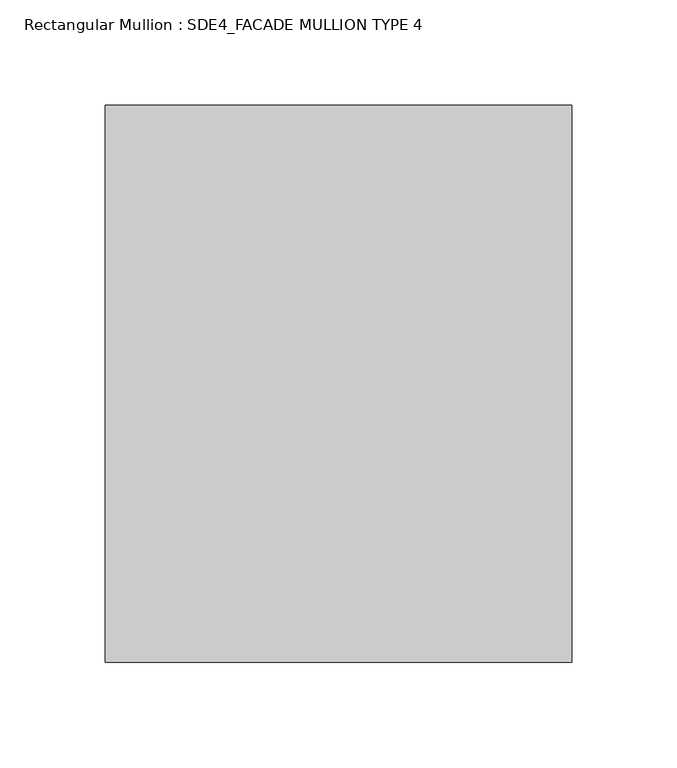
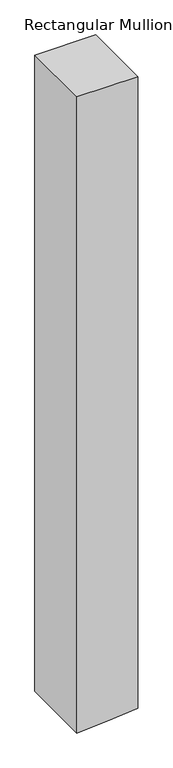
"""IFC4 building model written with IfcOpenShell, lengths in millimetres: member geometry, Rectangular Mullion : SDE4_FACADE MULLION TYPE 4."""

import ifcopenshell
import ifcopenshell.guid

model = None  # the IFC model being written
_history = None  # IfcOwnerHistory: only IFC2X3 demands one
_inside = {}  # id of a spatial element -> (the spatial element, [elements in it])
_under = {}  # id of a project, library or spatial element -> (it, [spatial elements below it])
_declared = {}  # id of a project -> (the project, [libraries it declares])
_typed = {}  # id of a type object -> (the type object, [elements of that type])
_made_of = {}  # id of a material, layer set ... -> (it, [elements and type objects made of it])


def new_model(schema):
    """Start an empty IFC model of exactly this schema.

    Asked for "IFC4X3", IfcOpenShell would pick the latest addendum, in which some entities
    have other attributes; the version numbers below select the first issue.
    IFC2X3 requires an IfcOwnerHistory on every rooted entity: one is made here for all.
    """
    global model, _history
    if schema == "IFC4X3":
        model = ifcopenshell.file(schema_version=(4, 3, 0, 0))
    else:
        model = ifcopenshell.file(schema=schema)
    _inside.clear()
    _under.clear()
    _declared.clear()
    _typed.clear()
    _made_of.clear()
    _history = None
    if model.schema == "IFC2X3":
        org = make("IfcOrganization", Name="unknown")
        user = make(
            "IfcPersonAndOrganization",
            ThePerson=make("IfcPerson", FamilyName="unknown"),
            TheOrganization=org,
        )
        app = make(
            "IfcApplication",
            ApplicationDeveloper=org,
            Version="unknown",
            ApplicationFullName="unknown",
            ApplicationIdentifier="unknown",
        )
        _history = make(
            "IfcOwnerHistory",
            OwningUser=user,
            OwningApplication=app,
            ChangeAction="ADDED",
            CreationDate=0,
        )
    return model


def make(cls, **values):
    """One entity of the class cls with the attributes given. An attribute that is None is left unset."""
    return model.create_entity(
        cls, **{name: value for name, value in values.items() if value is not None}
    )


def rooted(cls, **values):
    """An entity with a GlobalId (a new one), such as an element, a storey or a relation."""
    return make(cls, GlobalId=ifcopenshell.guid.new(), OwnerHistory=_history, **values)


def si_unit(unit_type, name, prefix=None):
    """IfcSIUnit, for example si_unit("LENGTHUNIT", "METRE", prefix="MILLI")."""
    return make("IfcSIUnit", UnitType=unit_type, Prefix=prefix, Name=name)


def assignment(units):
    """IfcUnitAssignment: the units of a project."""
    return None if units is None else make("IfcUnitAssignment", Units=units)


def point(xyz):
    """IfcCartesianPoint."""
    return None if xyz is None else make("IfcCartesianPoint", Coordinates=xyz)


def direction(xyz):
    """IfcDirection."""
    return None if xyz is None else make("IfcDirection", DirectionRatios=xyz)


def frame(location, z_axis=None, x_axis=None):
    """IfcAxis2Placement3D, a coordinate frame: its origin and axes. An axis left out is left unset."""
    return make(
        "IfcAxis2Placement3D",
        Location=point(location),
        Axis=direction(z_axis),
        RefDirection=direction(x_axis),
    )


def origin():
    """The frame at (0, 0, 0) with its axes left unset."""
    return frame((0.0, 0.0, 0.0))


def place(relative_to, where):
    """IfcLocalPlacement: puts the frame where relative to a parent placement (None: the world)."""
    return make(
        "IfcLocalPlacement", PlacementRelTo=relative_to, RelativePlacement=where
    )


def context(
    kind, dimensions, precision=None, world=None, true_north=None, identifier=None
):
    """IfcGeometricRepresentationContext, for example the 3D "Model" context."""
    return make(
        "IfcGeometricRepresentationContext",
        ContextIdentifier=identifier,
        ContextType=kind,
        CoordinateSpaceDimension=dimensions,
        Precision=precision,
        WorldCoordinateSystem=world,
        TrueNorth=true_north,
    )


def project(units=None, contexts=None):
    """IfcProject with its units and contexts."""
    return rooted(
        "IfcProject",
        Name="project",
        RepresentationContexts=contexts,
        UnitsInContext=assignment(units),
    )


def spatial(cls, under=None, at=None, **own):
    """A site, building, storey or space (cls), placed at a placement, below another one or the project."""
    s = rooted(cls, ObjectPlacement=at, **own)
    if under is not None:
        _under.setdefault(under.id(), (under, []))[1].append(s)
    return s


def polyline(points):
    """IfcPolyline through the points."""
    return make("IfcPolyline", Points=[point(p) for p in points])


def outline(outer, holes=None, kind="AREA"):
    """IfcArbitraryClosedProfileDef: a profile drawn as a closed curve; with holes, ...WithVoids."""
    if holes is None:
        return make("IfcArbitraryClosedProfileDef", ProfileType=kind, OuterCurve=outer)
    return make(
        "IfcArbitraryProfileDefWithVoids",
        ProfileType=kind,
        OuterCurve=outer,
        InnerCurves=holes,
    )


def extrude(swept, where, along, depth):
    """IfcExtrudedAreaSolid: the profile swept, set in the frame where, extruded along a direction by depth."""
    return make(
        "IfcExtrudedAreaSolid",
        SweptArea=swept,
        Position=where,
        ExtrudedDirection=direction(along),
        Depth=depth,
    )


def shape(context_of_items, identifier, shape_type, items):
    """IfcShapeRepresentation: the items that make up one representation, for example the "Body"."""
    return make(
        "IfcShapeRepresentation",
        ContextOfItems=context_of_items,
        RepresentationIdentifier=identifier,
        RepresentationType=shape_type,
        Items=items,
    )


def source(mapping_origin, context_of_items, identifier, shape_type, items):
    """IfcRepresentationMap: a shape defined once, which mapped items show again and again."""
    return make(
        "IfcRepresentationMap",
        MappingOrigin=mapping_origin,
        MappedRepresentation=shape(context_of_items, identifier, shape_type, items),
    )


def transform(
    local_origin,
    x_axis=None,
    y_axis=None,
    z_axis=None,
    scale=None,
    scale2=None,
    scale3=None,
    uniform=True,
):
    """IfcCartesianTransformationOperator3D, or its non-uniform kind. x_axis, y_axis, z_axis: its Axis1, 2, 3."""
    if uniform:
        return make(
            "IfcCartesianTransformationOperator3D",
            Axis1=direction(x_axis),
            Axis2=direction(y_axis),
            LocalOrigin=point(local_origin),
            Scale=scale,
            Axis3=direction(z_axis),
        )
    return make(
        "IfcCartesianTransformationOperator3DnonUniform",
        Axis1=direction(x_axis),
        Axis2=direction(y_axis),
        LocalOrigin=point(local_origin),
        Scale=scale,
        Axis3=direction(z_axis),
        Scale2=scale2,
        Scale3=scale3,
    )


def mapped(mapping_source, mapping_target):
    """IfcMappedItem: shows the shape of a source again, moved by a transform."""
    return make(
        "IfcMappedItem", MappingSource=mapping_source, MappingTarget=mapping_target
    )


def made_of(thing, what):
    """Note that an element or type object is made of a material, layer set ...; save() writes the relation."""
    if what is not None:
        _made_of.setdefault(what.id(), (what, []))[1].append(thing)
    return thing


def element(
    cls,
    number,
    at=None,
    inside=None,
    cuts=None,
    type_object=None,
    material=None,
    context=None,
    identifier="Body",
    shape_type=None,
    held_by="IfcProductDefinitionShape",
    body=None,
    shapes=None,
    **own,
):
    """One element of the class cls, such as IfcWall. Its Tag is "e" and its number.

    at: its placement. inside: the storey or other place that contains it. cuts: it is an
    opening in that element (IfcRelVoidsElement). A single representation is given by context,
    identifier, shape_type and body (its items); several are given by shapes. held_by: the class
    of the entity that holds the representations. save() writes the other relations.
    """
    e = rooted(cls, Tag="e%d" % number, ObjectPlacement=at, **own)
    if body is not None:
        shapes = [shape(context, identifier, shape_type, body)]
    if shapes is not None:
        e.Representation = make(held_by, Representations=shapes)
    if inside is not None:
        _inside.setdefault(inside.id(), (inside, []))[1].append(e)
    if cuts is not None:
        rooted(
            "IfcRelVoidsElement", RelatingBuildingElement=cuts, RelatedOpeningElement=e
        )
    if type_object is not None:
        _typed.setdefault(type_object.id(), (type_object, []))[1].append(e)
    return made_of(e, material)


def aggregate(whole, parts):
    """IfcRelAggregates: a whole, such as a stair, and the parts it consists of."""
    return rooted("IfcRelAggregates", RelatingObject=whole, RelatedObjects=parts)


def save(model, path):
    """Write the relations noted so far, then the file.

    IfcRelAggregates (storeys below a building ...), IfcRelContainedInSpatialStructure (elements
    in a storey), IfcRelDefinesByType, IfcRelAssociatesMaterial and IfcRelDeclares: one each for
    every whole, place, type object, material and project.
    """
    for whole, parts in _under.values():
        aggregate(whole, parts)
    for where, things in _inside.values():
        rooted(
            "IfcRelContainedInSpatialStructure",
            RelatedElements=things,
            RelatingStructure=where,
        )
    for kind, things in _typed.values():
        rooted("IfcRelDefinesByType", RelatedObjects=things, RelatingType=kind)
    for what, things in _made_of.values():
        rooted("IfcRelAssociatesMaterial", RelatedObjects=things, RelatingMaterial=what)
    for by, libraries in _declared.values():
        rooted("IfcRelDeclares", RelatingContext=by, RelatedDefinitions=libraries)
    model.write(path)


def rectangular_mullion_sde4_facade_mullion_type_4_76e9a99e(model_context):
    return source(origin(), model_context, "Body", "SweptSolid", [
        extrude(outline(polyline([(0.0, 111.0), (0.0, -111.0), (-2449.0276558, -111.0), (-2440.755216, -3.056508), (-2432.0142943, 111.0), (0.0, 111.0)])), frame((0.0, -132.5, 0.0), z_axis=(0.0, 1.0, 0.0), x_axis=(0.0, 0.0, 1.0)), (0.0, 0.0, 1.0), 265.0),
    ])


if __name__ == "__main__":
    model = new_model("IFC4")
    model_context = context("Model", 3, world=origin())
    ifc_project = project(units=[si_unit("LENGTHUNIT", "METRE", prefix="MILLI")], contexts=[model_context])
    site = spatial("IfcSite", under=ifc_project)
    building = spatial("IfcBuilding", under=site)
    placement = place(None, origin())
    rectangular_mullion_sde4_facade_mullion_type_4_shape = rectangular_mullion_sde4_facade_mullion_type_4_76e9a99e(model_context)
    element("IfcMember", 1, ObjectType="Rectangular Mullion : SDE4_FACADE MULLION TYPE 4", at=placement, inside=building, context=model_context, shape_type="MappedRepresentation", body=[
        mapped(rectangular_mullion_sde4_facade_mullion_type_4_shape, transform((0.0, 0.0, 0.0), x_axis=(1.0, 0.0, 0.0), y_axis=(0.0, 1.0, 0.0), z_axis=(0.0, 0.0, 1.0))),
    ])
    save(model, "model.ifc")

# Revit data of these elements
# Type "Rectangular Mullion : SDE4_FACADE MULLION TYPE 4"
#   built-in parameter 1007322 = 0.869423 (stored number, unit not read)
#   built-in parameter 1007321 = 0.364173 (stored number, unit not read)
#   built-in parameter 1007320 = 0.364173 (stored number, unit not read)
